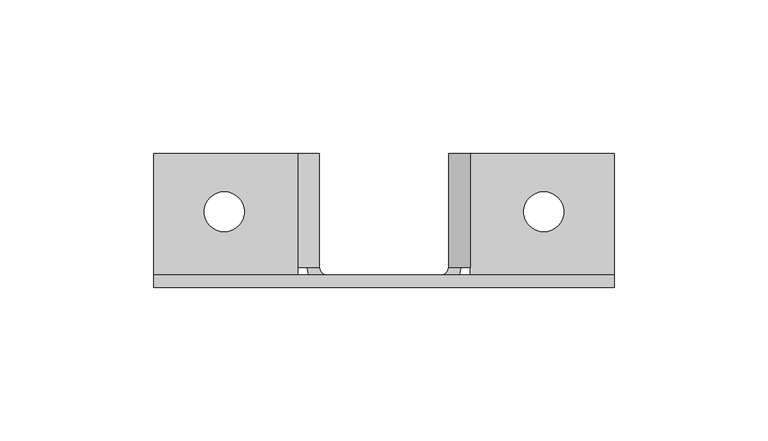
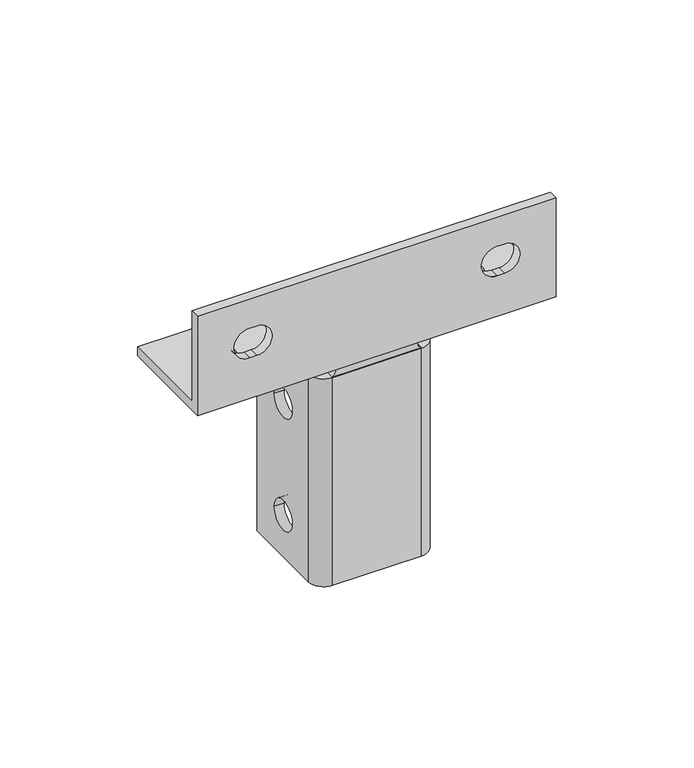
"""IFC4 building model written with IfcOpenShell, lengths in millimetres: proxy geometry, ❶ TN_Соединитель 3D Т-образный (сборка тип 1) : ❶ TN_Соединитель 3D Т-образный (сборка тип 1)."""

import ifcopenshell
import ifcopenshell.guid

model = None  # the IFC model being written
_history = None  # IfcOwnerHistory: only IFC2X3 demands one
_inside = {}  # id of a spatial element -> (the spatial element, [elements in it])
_under = {}  # id of a project, library or spatial element -> (it, [spatial elements below it])
_declared = {}  # id of a project -> (the project, [libraries it declares])
_typed = {}  # id of a type object -> (the type object, [elements of that type])
_made_of = {}  # id of a material, layer set ... -> (it, [elements and type objects made of it])


def new_model(schema):
    """Start an empty IFC model of exactly this schema.

    Asked for "IFC4X3", IfcOpenShell would pick the latest addendum, in which some entities
    have other attributes; the version numbers below select the first issue.
    IFC2X3 requires an IfcOwnerHistory on every rooted entity: one is made here for all.
    """
    global model, _history
    if schema == "IFC4X3":
        model = ifcopenshell.file(schema_version=(4, 3, 0, 0))
    else:
        model = ifcopenshell.file(schema=schema)
    _inside.clear()
    _under.clear()
    _declared.clear()
    _typed.clear()
    _made_of.clear()
    _history = None
    if model.schema == "IFC2X3":
        org = make("IfcOrganization", Name="unknown")
        user = make(
            "IfcPersonAndOrganization",
            ThePerson=make("IfcPerson", FamilyName="unknown"),
            TheOrganization=org,
        )
        app = make(
            "IfcApplication",
            ApplicationDeveloper=org,
            Version="unknown",
            ApplicationFullName="unknown",
            ApplicationIdentifier="unknown",
        )
        _history = make(
            "IfcOwnerHistory",
            OwningUser=user,
            OwningApplication=app,
            ChangeAction="ADDED",
            CreationDate=0,
        )
    return model


def make(cls, **values):
    """One entity of the class cls with the attributes given. An attribute that is None is left unset."""
    return model.create_entity(
        cls, **{name: value for name, value in values.items() if value is not None}
    )


def rooted(cls, **values):
    """An entity with a GlobalId (a new one), such as an element, a storey or a relation."""
    return make(cls, GlobalId=ifcopenshell.guid.new(), OwnerHistory=_history, **values)


def si_unit(unit_type, name, prefix=None):
    """IfcSIUnit, for example si_unit("LENGTHUNIT", "METRE", prefix="MILLI")."""
    return make("IfcSIUnit", UnitType=unit_type, Prefix=prefix, Name=name)


def assignment(units):
    """IfcUnitAssignment: the units of a project."""
    return None if units is None else make("IfcUnitAssignment", Units=units)


def point(xyz):
    """IfcCartesianPoint."""
    return None if xyz is None else make("IfcCartesianPoint", Coordinates=xyz)


def direction(xyz):
    """IfcDirection."""
    return None if xyz is None else make("IfcDirection", DirectionRatios=xyz)


def frame(location, z_axis=None, x_axis=None):
    """IfcAxis2Placement3D, a coordinate frame: its origin and axes. An axis left out is left unset."""
    return make(
        "IfcAxis2Placement3D",
        Location=point(location),
        Axis=direction(z_axis),
        RefDirection=direction(x_axis),
    )


def frame_2d(location, x_axis=None):
    """IfcAxis2Placement2D, a coordinate frame in the plane: its origin and x axis."""
    return make(
        "IfcAxis2Placement2D", Location=point(location), RefDirection=direction(x_axis)
    )


def origin():
    """The frame at (0, 0, 0) with its axes left unset."""
    return frame((0.0, 0.0, 0.0))


def place(relative_to, where):
    """IfcLocalPlacement: puts the frame where relative to a parent placement (None: the world)."""
    return make(
        "IfcLocalPlacement", PlacementRelTo=relative_to, RelativePlacement=where
    )


def context(
    kind, dimensions, precision=None, world=None, true_north=None, identifier=None
):
    """IfcGeometricRepresentationContext, for example the 3D "Model" context."""
    return make(
        "IfcGeometricRepresentationContext",
        ContextIdentifier=identifier,
        ContextType=kind,
        CoordinateSpaceDimension=dimensions,
        Precision=precision,
        WorldCoordinateSystem=world,
        TrueNorth=true_north,
    )


def project(units=None, contexts=None):
    """IfcProject with its units and contexts."""
    return rooted(
        "IfcProject",
        Name="project",
        RepresentationContexts=contexts,
        UnitsInContext=assignment(units),
    )


def spatial(cls, under=None, at=None, **own):
    """A site, building, storey or space (cls), placed at a placement, below another one or the project."""
    s = rooted(cls, ObjectPlacement=at, **own)
    if under is not None:
        _under.setdefault(under.id(), (under, []))[1].append(s)
    return s


def polyline(points):
    """IfcPolyline through the points."""
    return make("IfcPolyline", Points=[point(p) for p in points])


def circle_curve(where, radius):
    """IfcCircle in the frame where."""
    return make("IfcCircle", Position=where, Radius=radius)


def trimmed(basis, trim1, trim2, sense, master):
    """IfcTrimmedCurve: the piece of a basis curve between two trims."""
    return make(
        "IfcTrimmedCurve",
        BasisCurve=basis,
        Trim1=trim1,
        Trim2=trim2,
        SenseAgreement=sense,
        MasterRepresentation=master,
    )


def segment(curve, same_sense, transition):
    """IfcCompositeCurveSegment."""
    return make(
        "IfcCompositeCurveSegment",
        Transition=transition,
        SameSense=same_sense,
        ParentCurve=curve,
    )


def composite_curve(segments, self_intersect=None):
    """IfcCompositeCurve: segments joined end to end."""
    return make("IfcCompositeCurve", Segments=segments, SelfIntersect=self_intersect)


def outline(outer, holes=None, kind="AREA"):
    """IfcArbitraryClosedProfileDef: a profile drawn as a closed curve; with holes, ...WithVoids."""
    if holes is None:
        return make("IfcArbitraryClosedProfileDef", ProfileType=kind, OuterCurve=outer)
    return make(
        "IfcArbitraryProfileDefWithVoids",
        ProfileType=kind,
        OuterCurve=outer,
        InnerCurves=holes,
    )


def extrude(swept, where, along, depth):
    """IfcExtrudedAreaSolid: the profile swept, set in the frame where, extruded along a direction by depth."""
    return make(
        "IfcExtrudedAreaSolid",
        SweptArea=swept,
        Position=where,
        ExtrudedDirection=direction(along),
        Depth=depth,
    )


def shape(context_of_items, identifier, shape_type, items):
    """IfcShapeRepresentation: the items that make up one representation, for example the "Body"."""
    return make(
        "IfcShapeRepresentation",
        ContextOfItems=context_of_items,
        RepresentationIdentifier=identifier,
        RepresentationType=shape_type,
        Items=items,
    )


def source(mapping_origin, context_of_items, identifier, shape_type, items):
    """IfcRepresentationMap: a shape defined once, which mapped items show again and again."""
    return make(
        "IfcRepresentationMap",
        MappingOrigin=mapping_origin,
        MappedRepresentation=shape(context_of_items, identifier, shape_type, items),
    )


def transform(
    local_origin,
    x_axis=None,
    y_axis=None,
    z_axis=None,
    scale=None,
    scale2=None,
    scale3=None,
    uniform=True,
):
    """IfcCartesianTransformationOperator3D, or its non-uniform kind. x_axis, y_axis, z_axis: its Axis1, 2, 3."""
    if uniform:
        return make(
            "IfcCartesianTransformationOperator3D",
            Axis1=direction(x_axis),
            Axis2=direction(y_axis),
            LocalOrigin=point(local_origin),
            Scale=scale,
            Axis3=direction(z_axis),
        )
    return make(
        "IfcCartesianTransformationOperator3DnonUniform",
        Axis1=direction(x_axis),
        Axis2=direction(y_axis),
        LocalOrigin=point(local_origin),
        Scale=scale,
        Axis3=direction(z_axis),
        Scale2=scale2,
        Scale3=scale3,
    )


def mapped(mapping_source, mapping_target):
    """IfcMappedItem: shows the shape of a source again, moved by a transform."""
    return make(
        "IfcMappedItem", MappingSource=mapping_source, MappingTarget=mapping_target
    )


def made_of(thing, what):
    """Note that an element or type object is made of a material, layer set ...; save() writes the relation."""
    if what is not None:
        _made_of.setdefault(what.id(), (what, []))[1].append(thing)
    return thing


def element(
    cls,
    number,
    at=None,
    inside=None,
    cuts=None,
    type_object=None,
    material=None,
    context=None,
    identifier="Body",
    shape_type=None,
    held_by="IfcProductDefinitionShape",
    body=None,
    shapes=None,
    **own,
):
    """One element of the class cls, such as IfcWall. Its Tag is "e" and its number.

    at: its placement. inside: the storey or other place that contains it. cuts: it is an
    opening in that element (IfcRelVoidsElement). A single representation is given by context,
    identifier, shape_type and body (its items); several are given by shapes. held_by: the class
    of the entity that holds the representations. save() writes the other relations.
    """
    e = rooted(cls, Tag="e%d" % number, ObjectPlacement=at, **own)
    if body is not None:
        shapes = [shape(context, identifier, shape_type, body)]
    if shapes is not None:
        e.Representation = make(held_by, Representations=shapes)
    if inside is not None:
        _inside.setdefault(inside.id(), (inside, []))[1].append(e)
    if cuts is not None:
        rooted(
            "IfcRelVoidsElement", RelatingBuildingElement=cuts, RelatedOpeningElement=e
        )
    if type_object is not None:
        _typed.setdefault(type_object.id(), (type_object, []))[1].append(e)
    return made_of(e, material)


def aggregate(whole, parts):
    """IfcRelAggregates: a whole, such as a stair, and the parts it consists of."""
    return rooted("IfcRelAggregates", RelatingObject=whole, RelatedObjects=parts)


def save(model, path):
    """Write the relations noted so far, then the file.

    IfcRelAggregates (storeys below a building ...), IfcRelContainedInSpatialStructure (elements
    in a storey), IfcRelDefinesByType, IfcRelAssociatesMaterial and IfcRelDeclares: one each for
    every whole, place, type object, material and project.
    """
    for whole, parts in _under.values():
        aggregate(whole, parts)
    for where, things in _inside.values():
        rooted(
            "IfcRelContainedInSpatialStructure",
            RelatedElements=things,
            RelatingStructure=where,
        )
    for kind, things in _typed.values():
        rooted("IfcRelDefinesByType", RelatedObjects=things, RelatingType=kind)
    for what, things in _made_of.values():
        rooted("IfcRelAssociatesMaterial", RelatedObjects=things, RelatingMaterial=what)
    for by, libraries in _declared.values():
        rooted("IfcRelDeclares", RelatingContext=by, RelatedDefinitions=libraries)
    model.write(path)


def plane_surface(at):
    """IfcPlane: the flat surface through the origin of the frame at, square to its z axis."""
    return make("IfcPlane", Position=at)


def cylinder_surface(at, radius):
    """IfcCylindricalSurface: all points at the distance radius from the z axis of the frame at."""
    return make("IfcCylindricalSurface", Position=at, Radius=radius)


def revolved_surface(curve, axis_point, axis_direction):
    """IfcSurfaceOfRevolution: the curve turned about the line through axis_point along axis_direction."""
    return make(
        "IfcSurfaceOfRevolution",
        SweptCurve=make("IfcArbitraryOpenProfileDef", ProfileType="CURVE", Curve=curve),
        AxisPosition=make("IfcAxis1Placement", Location=point(axis_point), Axis=direction(axis_direction)),
    )


def advanced_brep(points, edges, surfaces, faces):
    """IfcAdvancedBrep: a solid bounded by faces that lie on surfaces and meet in shared edges.

    An edge is (start, end): straight between two places in points (the first is 0);
    or (start, end, curve); or (start, end, curve, False) where it runs against its curve.
    A face is (place in surfaces, loops), or (place, loops, False) where it looks against
    its surface's normal. A loop lists edges by number (the first is 1), with a minus sign
    where the edge is run from its end to its start. The first loop is the outer one.
    """
    corners = [point(p) for p in points]
    vertices = [make("IfcVertexPoint", VertexGeometry=c) for c in corners]
    made = []
    for start, end, *more in edges:
        made.append(
            make(
                "IfcEdgeCurve",
                EdgeStart=vertices[start],
                EdgeEnd=vertices[end],
                EdgeGeometry=more[0] if more else make("IfcPolyline", Points=[corners[start], corners[end]]),
                SameSense=more[1] if len(more) > 1 else True,
            )
        )
    hull = []
    for where, loops, *sense in faces:
        bounds = []
        for j, loop in enumerate(loops):
            ring = [make("IfcOrientedEdge", EdgeElement=made[abs(k) - 1], Orientation=k > 0) for k in loop]
            bounds.append(
                make(
                    "IfcFaceOuterBound" if j == 0 else "IfcFaceBound",
                    Bound=make("IfcEdgeLoop", EdgeList=ring),
                    Orientation=True,
                )
            )
        hull.append(make("IfcAdvancedFace", Bounds=bounds, FaceSurface=surfaces[where], SameSense=sense[0] if sense else True))
    return make("IfcAdvancedBrep", Outer=make("IfcClosedShell", CfsFaces=hull))


def generic_models_4b291d71(model_context):
    return source(origin(), model_context, "Body", "SolidModel", [
        advanced_brep(
        [(25.0, -18.1, 92.0), (28.0, -18.1, 95.0), (28.0, -18.1, 99.0), (21.0, -18.1, 92.0), (-21.0, -18.1, 92.0), (-28.0, -18.1, 99.0), (-28.0, -18.1, 95.0), (-25.0, -18.1, 92.0), (21.0, 19.0, 92.0), (28.0, 19.0, 99.0), (75.0, 19.0, 99.0), (75.0, 19.0, 95.0), (28.0, 19.0, 95.0), (25.0, 19.0, 92.0), (25.0, 19.0, 0.0), (21.0, 19.0, 0.0), (-25.0, 19.0, 92.0), (-28.0, 19.0, 95.0), (-75.0, 19.0, 95.0), (-75.0, 19.0, 99.0), (-28.0, 19.0, 99.0), (-21.0, 19.0, 92.0), (-21.0, 19.0, 0.0), (-25.0, 19.0, 0.0), (28.0, -20.6, 99.0), (75.0, -20.6, 99.0), (52.0, 6.5, 99.0), (52.0, -6.5, 99.0), (75.0, -20.6, 139.0), (75.0, -24.6, 139.0), (75.0, -24.6, 95.0), (75.0, -20.6, 95.0), (28.0, -20.6, 95.0), (52.0, -6.5, 95.0), (52.0, 6.5, 95.0), (-28.0, -20.6, 95.0), (-75.0, -24.6, 95.0), (-52.0, -6.5, 95.0), (-52.0, 6.5, 95.0), (-75.0, -24.6, 139.0), (-75.0, -20.6, 139.0), (-75.0, -20.6, 99.0), (-28.0, -20.6, 99.0), (-52.0, 6.5, 99.0), (-52.0, -6.5, 99.0), (53.4, -20.6, 126.0), (50.4, -20.6, 126.0), (50.4, -20.6, 113.0), (53.4, -20.6, 113.0), (-53.4, -20.6, 126.0), (-53.4, -20.6, 113.0), (-50.4, -20.6, 113.0), (-50.4, -20.6, 126.0), (50.4, -24.6, 126.0), (53.4, -24.6, 126.0), (53.4, -24.6, 113.0), (50.4, -24.6, 113.0), (-53.4, -24.6, 113.0), (-53.4, -24.6, 126.0), (-50.4, -24.6, 126.0), (-50.4, -24.6, 113.0), (-18.5, -24.6, 92.0), (18.5, -24.6, 92.0), (18.5, -20.6, 92.0), (-18.5, -20.6, 92.0), (-25.0, -18.1, 0.0), (-21.0, -18.1, 0.0), (-18.5, -20.6, 0.0), (18.5, -20.6, 0.0), (21.0, -18.1, 0.0), (25.0, -18.1, 0.0), (18.5, -24.6, 0.0), (-18.5, -24.6, 0.0), (25.0, 6.5, 18.5), (25.0, -6.5, 18.5), (25.0, 6.5, 68.5), (25.0, -6.5, 68.5), (21.0, -6.5, 18.5), (21.0, 6.5, 18.5), (21.0, -6.5, 68.5), (21.0, 6.5, 68.5), (-21.0, 6.5, 18.5), (-21.0, -6.5, 18.5), (-21.0, 6.5, 68.5), (-21.0, -6.5, 68.5), (-25.0, -6.5, 18.5), (-25.0, 6.5, 18.5), (-25.0, -6.5, 68.5), (-25.0, 6.5, 68.5)],
        [
            (0, 1, circle_curve(frame((28.0, -18.1, 92.0), z_axis=(0.0, 1.0, 0.0), x_axis=(-1.0, 0.0, 0.0)), 3.0)),
            (1, 2),
            (2, 3, circle_curve(frame((28.0, -18.1, 92.0), z_axis=(0.0, -1.0, 0.0), x_axis=(-1.0, 0.0, 0.0)), 7.0)),
            (3, 0),
            (4, 5, circle_curve(frame((-28.0, -18.1, 92.0), z_axis=(0.0, -1.0, 0.0), x_axis=(-1.0, 0.0, 0.0)), 7.0)),
            (5, 6),
            (6, 7, circle_curve(frame((-28.0, -18.1, 92.0), z_axis=(0.0, 1.0, 0.0), x_axis=(-1.0, 0.0, 0.0)), 3.0)),
            (7, 4),
            (8, 9, circle_curve(frame((28.0, 19.0, 92.0), z_axis=(0.0, 1.0, 0.0), x_axis=(-1.0, 0.0, 0.0)), 7.0)),
            (9, 10),
            (10, 11),
            (11, 12),
            (12, 13, circle_curve(frame((28.0, 19.0, 92.0), z_axis=(0.0, -1.0, 0.0), x_axis=(-1.0, 0.0, 0.0)), 3.0)),
            (13, 14),
            (14, 15),
            (15, 8),
            (16, 17, circle_curve(frame((-28.0, 19.0, 92.0), z_axis=(0.0, -1.0, 0.0), x_axis=(-1.0, 0.0, 0.0)), 3.0)),
            (17, 18),
            (18, 19),
            (19, 20),
            (20, 21, circle_curve(frame((-28.0, 19.0, 92.0), z_axis=(0.0, 1.0, 0.0), x_axis=(-1.0, 0.0, 0.0)), 7.0)),
            (21, 22),
            (22, 23),
            (23, 16),
            (2, 9),
            (8, 3),
            (2, 24),
            (24, 25),
            (25, 10),
            (26, 27, circle_curve(frame((52.0, 0.0, 99.0), z_axis=(0.0, 0.0, -1.0), x_axis=(0.0, -1.0, 0.0)), 6.5)),
            (27, 26, circle_curve(frame((52.0, 0.0, 99.0), z_axis=(0.0, 0.0, -1.0), x_axis=(0.0, -1.0, 0.0)), 6.5)),
            (25, 28),
            (28, 29),
            (29, 30),
            (30, 31),
            (31, 11),
            (31, 32),
            (32, 1),
            (1, 12),
            (33, 34, circle_curve(frame((52.0, 0.0, 95.0), z_axis=(0.0, 0.0, 1.0), x_axis=(0.0, -1.0, 0.0)), 6.5)),
            (34, 33, circle_curve(frame((52.0, 0.0, 95.0), z_axis=(0.0, 0.0, 1.0), x_axis=(0.0, -1.0, 0.0)), 6.5)),
            (0, 13),
            (6, 17),
            (16, 7),
            (6, 35),
            (35, 32),
            (30, 36),
            (36, 18),
            (37, 38, circle_curve(frame((-52.0, 0.0, 95.0), z_axis=(0.0, 0.0, 1.0), x_axis=(0.0, -1.0, 0.0)), 6.5)),
            (38, 37, circle_curve(frame((-52.0, 0.0, 95.0), z_axis=(0.0, 0.0, 1.0), x_axis=(0.0, -1.0, 0.0)), 6.5)),
            (36, 39),
            (39, 40),
            (40, 41),
            (41, 19),
            (41, 42),
            (42, 5),
            (5, 20),
            (43, 44, circle_curve(frame((-52.0, 0.0, 99.0), z_axis=(0.0, 0.0, -1.0), x_axis=(0.0, -1.0, 0.0)), 6.5)),
            (44, 43, circle_curve(frame((-52.0, 0.0, 99.0), z_axis=(0.0, 0.0, -1.0), x_axis=(0.0, -1.0, 0.0)), 6.5)),
            (4, 21),
            (37, 44),
            (43, 38),
            (33, 27),
            (26, 34),
            (28, 40),
            (39, 29),
            (24, 32),
            (35, 42),
            (45, 46),
            (46, 47, circle_curve(frame((50.4, -20.6, 119.5), z_axis=(0.0, -1.0, 0.0), x_axis=(1.0, 0.0, 0.0)), 6.5)),
            (47, 48),
            (48, 45, circle_curve(frame((53.4, -20.6, 119.5), z_axis=(0.0, -1.0, 0.0), x_axis=(1.0, 0.0, 0.0)), 6.5)),
            (49, 50, circle_curve(frame((-53.4, -20.6, 119.5), z_axis=(0.0, -1.0, 0.0), x_axis=(1.0, 0.0, 0.0)), 6.5)),
            (50, 51),
            (51, 52, circle_curve(frame((-50.4, -20.6, 119.5), z_axis=(0.0, -1.0, 0.0), x_axis=(1.0, 0.0, 0.0)), 6.5)),
            (52, 49),
            (53, 54),
            (54, 55, circle_curve(frame((53.4, -24.6, 119.5), z_axis=(0.0, 1.0, 0.0), x_axis=(1.0, 0.0, 0.0)), 6.5)),
            (55, 56),
            (56, 53, circle_curve(frame((50.4, -24.6, 119.5), z_axis=(0.0, 1.0, 0.0), x_axis=(1.0, 0.0, 0.0)), 6.5)),
            (57, 58, circle_curve(frame((-53.4, -24.6, 119.5), z_axis=(0.0, 1.0, 0.0), x_axis=(1.0, 0.0, 0.0)), 6.5)),
            (58, 59),
            (59, 60, circle_curve(frame((-50.4, -24.6, 119.5), z_axis=(0.0, 1.0, 0.0), x_axis=(1.0, 0.0, 0.0)), 6.5)),
            (60, 57),
            (53, 46),
            (45, 54),
            (56, 47),
            (55, 48),
            (57, 50),
            (49, 58),
            (60, 51),
            (59, 52),
            (7, 61, circle_curve(frame((-18.5, -18.1, 92.0), z_axis=(0.0, 0.0, 1.0), x_axis=(1.0, 0.0, 0.0)), 6.5)),
            (61, 62),
            (62, 0, circle_curve(frame((18.5, -18.1, 92.0), z_axis=(0.0, 0.0, 1.0), x_axis=(1.0, 0.0, 0.0)), 6.5)),
            (3, 63, circle_curve(frame((18.5, -18.1, 92.0), z_axis=(0.0, 0.0, -1.0), x_axis=(1.0, 0.0, 0.0)), 2.5)),
            (63, 64),
            (64, 4, circle_curve(frame((-18.5, -18.1, 92.0), z_axis=(0.0, 0.0, -1.0), x_axis=(1.0, 0.0, 0.0)), 2.5)),
            (65, 23),
            (22, 66),
            (66, 67, circle_curve(frame((-18.5, -18.1, 0.0), z_axis=(0.0, 0.0, 1.0), x_axis=(1.0, 0.0, 0.0)), 2.5)),
            (67, 68),
            (68, 69, circle_curve(frame((18.5, -18.1, 0.0), z_axis=(0.0, 0.0, 1.0), x_axis=(1.0, 0.0, 0.0)), 2.5)),
            (69, 15),
            (14, 70),
            (70, 71, circle_curve(frame((18.5, -18.1, 0.0), z_axis=(0.0, 0.0, -1.0), x_axis=(1.0, 0.0, 0.0)), 6.5)),
            (71, 72),
            (72, 65, circle_curve(frame((-18.5, -18.1, 0.0), z_axis=(0.0, 0.0, -1.0), x_axis=(1.0, 0.0, 0.0)), 6.5)),
            (61, 72),
            (71, 62),
            (0, 70),
            (73, 74, circle_curve(frame((25.0, 0.0, 18.5), z_axis=(-1.0, 0.0, 0.0), x_axis=(0.0, -1.0, 0.0)), 6.5)),
            (74, 73, circle_curve(frame((25.0, 0.0, 18.5), z_axis=(-1.0, 0.0, 0.0), x_axis=(0.0, -1.0, 0.0)), 6.5)),
            (75, 76, circle_curve(frame((25.0, 0.0, 68.5), z_axis=(-1.0, 0.0, 0.0), x_axis=(0.0, -1.0, 0.0)), 6.5)),
            (76, 75, circle_curve(frame((25.0, 0.0, 68.5), z_axis=(-1.0, 0.0, 0.0), x_axis=(0.0, -1.0, 0.0)), 6.5)),
            (69, 3),
            (77, 78, circle_curve(frame((21.0, 0.0, 18.5), z_axis=(1.0, 0.0, 0.0), x_axis=(0.0, -1.0, 0.0)), 6.5)),
            (78, 77, circle_curve(frame((21.0, 0.0, 18.5), z_axis=(1.0, 0.0, 0.0), x_axis=(0.0, -1.0, 0.0)), 6.5)),
            (79, 80, circle_curve(frame((21.0, 0.0, 68.5), z_axis=(1.0, 0.0, 0.0), x_axis=(0.0, -1.0, 0.0)), 6.5)),
            (80, 79, circle_curve(frame((21.0, 0.0, 68.5), z_axis=(1.0, 0.0, 0.0), x_axis=(0.0, -1.0, 0.0)), 6.5)),
            (63, 68),
            (67, 64),
            (4, 66),
            (81, 82, circle_curve(frame((-21.0, 0.0, 18.5), z_axis=(-1.0, 0.0, 0.0), x_axis=(0.0, -1.0, 0.0)), 6.5)),
            (82, 81, circle_curve(frame((-21.0, 0.0, 18.5), z_axis=(-1.0, 0.0, 0.0), x_axis=(0.0, -1.0, 0.0)), 6.5)),
            (83, 84, circle_curve(frame((-21.0, 0.0, 68.5), z_axis=(-1.0, 0.0, 0.0), x_axis=(0.0, -1.0, 0.0)), 6.5)),
            (84, 83, circle_curve(frame((-21.0, 0.0, 68.5), z_axis=(-1.0, 0.0, 0.0), x_axis=(0.0, -1.0, 0.0)), 6.5)),
            (65, 7),
            (85, 86, circle_curve(frame((-25.0, 0.0, 18.5), z_axis=(1.0, 0.0, 0.0), x_axis=(0.0, -1.0, 0.0)), 6.5)),
            (86, 85, circle_curve(frame((-25.0, 0.0, 18.5), z_axis=(1.0, 0.0, 0.0), x_axis=(0.0, -1.0, 0.0)), 6.5)),
            (87, 88, circle_curve(frame((-25.0, 0.0, 68.5), z_axis=(1.0, 0.0, 0.0), x_axis=(0.0, -1.0, 0.0)), 6.5)),
            (88, 87, circle_curve(frame((-25.0, 0.0, 68.5), z_axis=(1.0, 0.0, 0.0), x_axis=(0.0, -1.0, 0.0)), 6.5)),
            (73, 78),
            (77, 74),
            (81, 86),
            (85, 82),
            (75, 80),
            (79, 76),
            (83, 88),
            (87, 84),
        ],
        [
            plane_surface(frame((21.0, -18.1, 92.0), z_axis=(0.0, -1.0, 0.0), x_axis=(1.0, 0.0, 0.0))),
            plane_surface(frame((21.0, 19.0, 92.0), z_axis=(0.0, 1.0, 0.0), x_axis=(-1.0, 0.0, 0.0))),
            cylinder_surface(frame((28.0, -18.1, 92.0), z_axis=(0.0, 1.0, 0.0), x_axis=(-1.0, 0.0, 0.0)), 7.0),
            plane_surface(frame((28.0, 19.0, 99.0), z_axis=(0.0, 0.0, 1.0), x_axis=(0.0, -1.0, 0.0))),
            plane_surface(frame((75.0, 19.0, 99.0), z_axis=(1.0, 0.0, 0.0), x_axis=(0.0, -1.0, 0.0))),
            plane_surface(frame((75.0, 19.0, 95.0), z_axis=(0.0, 0.0, -1.0), x_axis=(0.0, -1.0, 0.0))),
            revolved_surface(polyline([(25.0, -18.1, 92.0), (25.0, 19.0, 92.0)]), (28.0, -18.1, 92.0), (0.0, -1.0, 0.0)),
            revolved_surface(polyline([(-31.0, -18.1, 92.0), (-31.0, 19.0, 92.0)]), (-28.0, 19.0, 92.0), (0.0, -1.0, 0.0)),
            plane_surface(frame((-28.0, 19.0, 95.0), z_axis=(0.0, 0.0, -1.0), x_axis=(0.0, -1.0, 0.0))),
            plane_surface(frame((-75.0, 19.0, 95.0), z_axis=(-1.0, 0.0, 0.0), x_axis=(0.0, -1.0, 0.0))),
            plane_surface(frame((-75.0, 19.0, 99.0), z_axis=(0.0, 0.0, 1.0), x_axis=(0.0, -1.0, 0.0))),
            cylinder_surface(frame((-28.0, 19.0, 92.0), z_axis=(0.0, 1.0, 0.0), x_axis=(-1.0, 0.0, 0.0)), 7.0),
            revolved_surface(polyline([(-52.0, -6.5, 95.0), (-52.0, -6.5, 99.0)]), (-52.0, 0.0, 99.0), (0.0, 0.0, -1.0)),
            revolved_surface(polyline([(52.0, -6.5, 95.0), (52.0, -6.5, 99.0)]), (52.0, 0.0, 99.0), (0.0, 0.0, -1.0)),
            plane_surface(frame((-75.0, -20.6, 139.0), z_axis=(0.0, 0.0, 1.0), x_axis=(-1.0, 0.0, 0.0))),
            plane_surface(frame((75.0, -20.6, 139.0), z_axis=(0.0, 1.0, 0.0), x_axis=(0.0, 0.0, -1.0))),
            plane_surface(frame((-75.0, -24.6, 139.0), z_axis=(0.0, -1.0, 0.0), x_axis=(0.0, 0.0, -1.0))),
            plane_surface(frame((53.4, -24.6, 126.0), z_axis=(0.0, 0.0, -1.0), x_axis=(0.0, 1.0, 0.0))),
            revolved_surface(polyline([(56.9, -24.6, 119.5), (56.9, -20.6, 119.5)]), (50.4, -21.0, 119.5), (0.0, -1.0, 0.0)),
            plane_surface(frame((50.4, -24.6, 113.0), z_axis=(0.0, 0.0, 1.0), x_axis=(0.0, 1.0, 0.0))),
            revolved_surface(polyline([(59.9, -24.6, 119.5), (59.9, -20.6, 119.5)]), (53.4, -21.0, 119.5), (0.0, -1.0, 0.0)),
            revolved_surface(polyline([(-46.9, -24.6, 119.5), (-46.9, -20.6, 119.5)]), (-53.4, -21.0, 119.5), (0.0, -1.0, 0.0)),
            plane_surface(frame((-53.4, -24.6, 113.0), z_axis=(0.0, 0.0, 1.0), x_axis=(0.0, 1.0, 0.0))),
            revolved_surface(polyline([(-43.9, -24.6, 119.5), (-43.9, -20.6, 119.5)]), (-50.4, -21.0, 119.5), (0.0, -1.0, 0.0)),
            plane_surface(frame((-50.4, -24.6, 126.0), z_axis=(0.0, 0.0, -1.0), x_axis=(0.0, 1.0, 0.0))),
            plane_surface(frame((-28.0, -18.1, 99.0), z_axis=(1.0, 0.0, 0.0), x_axis=(0.0, -1.0, 0.0))),
            plane_surface(frame((28.0, -18.1, 95.0), z_axis=(-1.0, 0.0, 0.0), x_axis=(0.0, -1.0, 0.0))),
            plane_surface(frame((-12.0, -18.1, 92.0), z_axis=(0.0, 0.0, 1.0), x_axis=(0.0, 1.0, 0.0))),
            plane_surface(frame((-12.0, -18.1, 0.0), z_axis=(0.0, 0.0, -1.0), x_axis=(0.0, -1.0, 0.0))),
            plane_surface(frame((-18.5, -24.6, 92.0), z_axis=(0.0, -1.0, 0.0), x_axis=(0.0, 0.0, -1.0))),
            plane_surface(frame((25.0, -18.1, 92.0), z_axis=(1.0, 0.0, 0.0), x_axis=(0.0, 0.0, -1.0))),
            plane_surface(frame((21.0, 19.0, 92.0), z_axis=(-1.0, 0.0, 0.0), x_axis=(0.0, 0.0, -1.0))),
            plane_surface(frame((18.5, -20.6, 92.0), z_axis=(0.0, 1.0, 0.0), x_axis=(0.0, 0.0, -1.0))),
            plane_surface(frame((-21.0, -18.1, 92.0), z_axis=(1.0, 0.0, 0.0), x_axis=(0.0, 0.0, -1.0))),
            plane_surface(frame((-25.0, 19.0, 92.0), z_axis=(-1.0, 0.0, 0.0), x_axis=(0.0, 0.0, -1.0))),
            cylinder_surface(frame((-18.5, -18.1, 0.0), z_axis=(0.0, 0.0, 1.0), x_axis=(1.0, 0.0, 0.0)), 6.5),
            cylinder_surface(frame((18.5, -18.1, 0.0), z_axis=(0.0, 0.0, 1.0), x_axis=(1.0, 0.0, 0.0)), 6.5),
            revolved_surface(polyline([(21.0, -18.1, 0.0), (21.0, -18.1, 92.0)]), (18.5, -18.1, 0.0), (0.0, 0.0, -1.0)),
            revolved_surface(polyline([(-16.0, -18.1, 0.0), (-16.0, -18.1, 92.0)]), (-18.5, -18.1, 0.0), (0.0, 0.0, -1.0)),
            revolved_surface(polyline([(21.0, -6.5, 18.5), (25.0, -6.5, 18.5)]), (25.0, 0.0, 18.5), (-1.0, 0.0, 0.0)),
            revolved_surface(polyline([(-25.0, -6.5, 18.5), (-21.0, -6.5, 18.5)]), (25.0, 0.0, 18.5), (-1.0, 0.0, 0.0)),
            revolved_surface(polyline([(21.0, -6.5, 68.5), (25.0, -6.5, 68.5)]), (0.0, 0.0, 68.5), (-1.0, 0.0, 0.0)),
            revolved_surface(polyline([(-25.0, -6.5, 68.5), (-21.0, -6.5, 68.5)]), (0.0, 0.0, 68.5), (-1.0, 0.0, 0.0)),
        ],
        [
            (0, [[1, 2, 3, 4]]),
            (0, [[5, 6, 7, 8]]),
            (1, [[9, 10, 11, 12, 13, 14, 15, 16]]),
            (1, [[17, 18, 19, 20, 21, 22, 23, 24]]),
            (2, [[-3, 25, -9, 26]]),
            (3, [[-10, -25, 27, 28, 29], [30, 31]]),
            (4, [[-11, -29, 32, 33, 34, 35, 36]]),
            (5, [[-12, -36, 37, 38, 39], [40, 41]]),
            (6, [[-1, 42, -13, -39]]),
            (7, [[-7, 43, -17, 44]]),
            (8, [[-18, -43, 45, 46, -37, -35, 47, 48], [49, 50]]),
            (9, [[-19, -48, 51, 52, 53, 54]]),
            (10, [[-20, -54, 55, 56, 57], [58, 59]]),
            (11, [[-5, 60, -21, -57]]),
            (12, [[61, -58, 62, -49]]),
            (12, [[-61, -50, -62, -59]]),
            (13, [[63, -30, 64, -40]]),
            (13, [[-63, -41, -64, -31]]),
            (14, [[65, -52, 66, -33]]),
            (15, [[-65, -32, -28, 67, -46, 68, -55, -53], [69, 70, 71, 72], [73, 74, 75, 76]]),
            (16, [[-66, -51, -47, -34], [77, 78, 79, 80], [81, 82, 83, 84]]),
            (17, [[85, -69, 86, -77]]),
            (18, [[-85, -80, 87, -70]]),
            (19, [[-87, -79, 88, -71]]),
            (20, [[-86, -72, -88, -78]]),
            (21, [[89, -73, 90, -81]]),
            (22, [[-89, -84, 91, -74]]),
            (23, [[-91, -83, 92, -75]]),
            (24, [[-90, -76, -92, -82]]),
            (25, [[-45, -6, -56, -68]]),
            (26, [[-38, -67, -27, -2]]),
            (27, [[93, 94, 95, -4, 96, 97, 98, -8]]),
            (28, [[99, -23, 100, 101, 102, 103, 104, -15, 105, 106, 107, 108]]),
            (29, [[-94, 109, -107, 110]]),
            (30, [[-105, -14, -42, 111], [112, 113], [114, 115]]),
            (31, [[-104, 116, -26, -16], [117, 118], [119, 120]]),
            (32, [[-97, 121, -102, 122]]),
            (33, [[-100, -22, -60, 123], [124, 125], [126, 127]]),
            (34, [[-99, 128, -44, -24], [129, 130], [131, 132]]),
            (35, [[-93, -128, -108, -109]]),
            (36, [[-95, -110, -106, -111]]),
            (37, [[-96, -116, -103, -121]]),
            (38, [[-98, -122, -101, -123]]),
            (39, [[133, -117, 134, -112]]),
            (40, [[135, -129, 136, -124]]),
            (39, [[-133, -113, -134, -118]]),
            (40, [[-135, -125, -136, -130]]),
            (41, [[137, -119, 138, -114]]),
            (42, [[139, -131, 140, -126]]),
            (41, [[-137, -115, -138, -120]]),
            (42, [[-139, -127, -140, -132]]),
        ],
    ),
        extrude(outline(composite_curve([segment(trimmed(circle_curve(frame_2d((95.0, -20.0)), 3.0), [point((95.0, -17.0))], [point((92.0, -20.0))], True, "CARTESIAN"), True, "CONTINUOUS"), segment(polyline([(92.0, -20.0), (92.0, 20.0)]), True, "CONTINUOUS"), segment(trimmed(circle_curve(frame_2d((95.0, 20.0)), 3.0), [point((92.0, 20.0))], [point((95.0, 17.0))], True, "CARTESIAN"), True, "CONTINUOUS"), segment(polyline([(95.0, 17.0), (95.0, 0.0), (95.0, -17.0)]), True, "CONTINUOUS")], self_intersect=False)), frame((0.0, -24.6, 0.0), z_axis=(0.0, 1.0, 0.0), x_axis=(0.0, 0.0, 1.0)), (0.0, 0.0, 1.0), 4.0),
    ])


if __name__ == "__main__":
    model = new_model("IFC4")
    model_context = context("Model", 3, world=origin())
    ifc_project = project(units=[si_unit("LENGTHUNIT", "METRE", prefix="MILLI")], contexts=[model_context])
    site = spatial("IfcSite", under=ifc_project)
    building = spatial("IfcBuilding", under=site)
    placement = place(None, origin())
    generic_models_shape = generic_models_4b291d71(model_context)
    element("IfcBuildingElementProxy", 1, Name="❶ TN_Соединитель 3D Т-образный (сборка тип 1) : ❶ TN_Соединитель 3D Т-образный (сборка тип 1)", ObjectType="❶ TN_Соединитель 3D Т-образный (сборка тип 1) : ❶ TN_Соединитель 3D Т-образный (сборка тип 1)", at=placement, inside=building, context=model_context, shape_type="MappedRepresentation", body=[
        mapped(generic_models_shape, transform((0.0, 0.0, 0.0), x_axis=(1.0, 0.0, 0.0), y_axis=(0.0, 1.0, 0.0), z_axis=(0.0, 0.0, 1.0))),
    ])
    save(model, "model.ifc")

# Revit data of these elements
# Type "❶ TN_Соединитель 3D Т-образный (сборка тип 1) : ❶ TN_Соединитель 3D Т-образный (сборка тип 1)"
#   Description = "Элемент для создания пространственных конструкций из профилей."
#   Manufacturer = "ТехноНИКОЛЬ"
#   Model = "Комплектующие к опорам"
#   URL = "https://nav.tn.ru/knowledge-base/polimernye-membrany/opory-pod-oborudovanie-na-ploskoy-krovle/?sphrase_id=266812"
#   ADSK_Обозначение = "ТехноНИКОЛЬ"
#   ADSK_Наименование краткое = "3D T 38-41 4F10"
#   ADSK_Наименование = "Соединитель 3D Т-образный 38-41 4F10"
#   ADSK_Масса_Текст = ""
#   ADSK_Марка = "3D T 38-41 4F10"
#   ADSK_Код изделия = "660821"
#   ADSK_Завод-изготовитель = "ТехноНИКОЛЬ"
#   ADSK_Единица измерения = "шт."
#   ADSK_Группирование = "Комплектующие к опорам"
#   ADSK_URL страницы изделия = "https://nav.tn.ru/knowledge-base/polimernye-membrany/opory-pod-oborudovanie-na-ploskoy-krovle/?sphrase_id=266812"
#   ADSK_URL документации изделия = ""
#   ADSK_Количество = 1
#   ADSK_Материал = TN_СтальГальванизированная_Серый
#   Default Elevation = 0
# Element 1 (IfcBuildingElementProxy, "❶ TN_Соединитель 3D Т-образный (сборка тип 1) : ❶ TN_Соединитель 3D Т-образный (сборка тип 1)")
#   Materials on its faces: "TN_СтальГальванизированная_Серый"
# Materials
#   "TN_СтальГальванизированная_Серый": class "Типовые", colour RGB 206 210 213, transparency 0, Cost = 0
